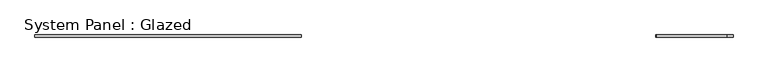
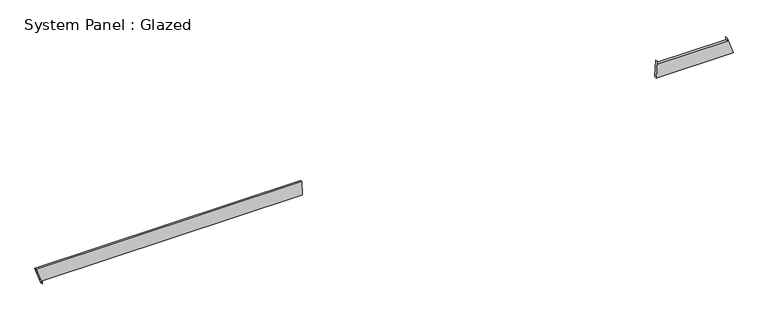
"""IFC4 building model written with IfcOpenShell, lengths in millimetres: plate geometry, System Panel : Glazed."""

from ifc_helpers import new_model, si_unit, frame, origin, place, context, project, spatial, polyline, outline, extrude, source, transform, mapped, element, save


def system_panel_glazed_62bd49df(model_context):
    return source(origin(), model_context, "Body", "SweptSolid", [
        extrude(outline(polyline([(35.3553391, 3137.6400042), (35.3553391, 4027.6365543), (235.670353, 3958.7537794), (200.315014, 3958.7544121), (200.3005351, 3149.6593447), (235.6558742, 3149.6587121), (35.3553391, 3137.6400042)])), frame((0.0, -49.5, 0.0), z_axis=(0.0, 1.0, 0.0), x_axis=(0.0, 0.0, 1.0)), (0.0, 0.0, 1.0), 25.0),
        extrude(outline(polyline([(0.0, -3958.4083386), (35.3553391, -3958.4083386), (35.3553391, -952.2431846), (200.2270781, -955.2036459), (200.1720966, -4027.6365543), (0.0, -3958.4083386)])), frame((0.0, -49.5, 0.0), z_axis=(0.0, 1.0, 0.0), x_axis=(0.0, 0.0, 1.0)), (0.0, 0.0, 1.0), 25.0),
    ])


if __name__ == "__main__":
    model = new_model("IFC4")
    model_context = context("Model", 3, world=origin())
    ifc_project = project(units=[si_unit("LENGTHUNIT", "METRE", prefix="MILLI")], contexts=[model_context])
    site = spatial("IfcSite", under=ifc_project)
    building = spatial("IfcBuilding", under=site)
    placement = place(None, origin())
    system_panel_glazed_shape = system_panel_glazed_62bd49df(model_context)
    element("IfcPlate", 1, ObjectType="System Panel : Glazed", at=placement, inside=building, context=model_context, shape_type="MappedRepresentation", body=[
        mapped(system_panel_glazed_shape, transform((0.0, 0.0, 0.0), x_axis=(1.0, 0.0, 0.0), y_axis=(0.0, 1.0, 0.0), z_axis=(0.0, 0.0, 1.0))),
    ])
    save(model, "model.ifc")

# Revit data of these elements
# Element 1 (IfcPlate, "System Panel : Glazed")
#   Materials on its faces: "Glass"
# Materials
#   "Glass": class "Glass", colour RGB 218 227 224, transparency 0.85, Description = "Soda Lime Glass", Cost = 0
